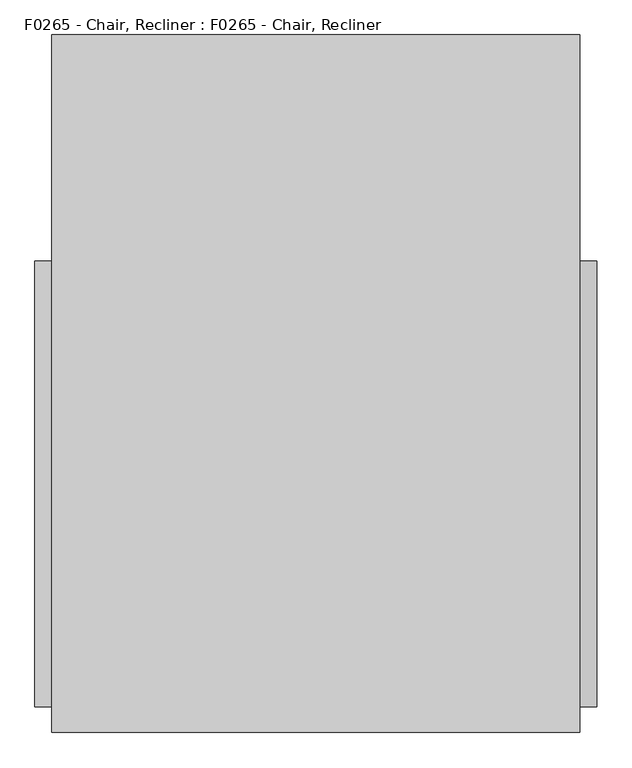
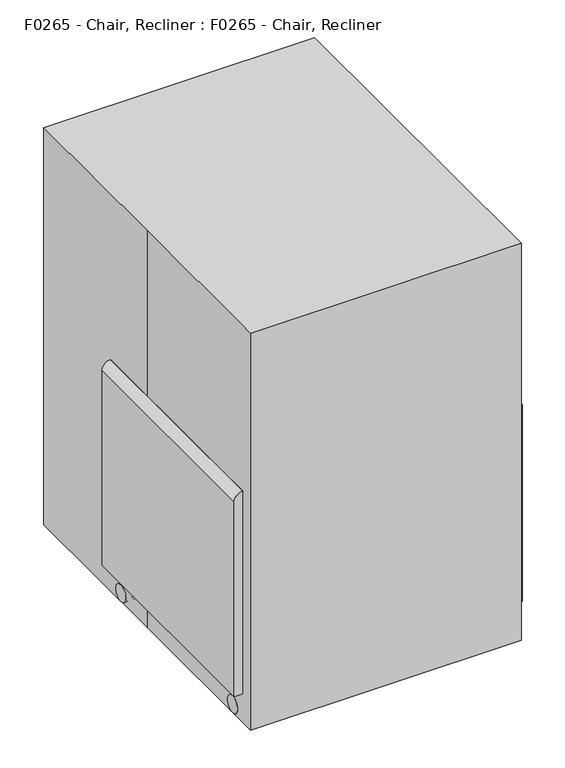
"""IFC4 building model written with IfcOpenShell, lengths in millimetres: proxy geometry, F0265 - Chair, Recliner : F0265 - Chair, Recliner."""

from ifc_helpers import new_model, si_unit, point, frame, frame_2d, origin, origin_with_axes, place, context, project, spatial, polyline, circle_curve, trimmed, segment, composite_curve, outline, extrude, source, transform, mapped, element, save


def f0265_chair_recliner_f0265_chair_recliner_6c0222d9(model_context):
    return source(origin(), model_context, "Body", "SweptSolid", [
        extrude(outline(composite_curve([segment(trimmed(circle_curve(frame_2d((131.7625, 25.4)), 25.4), [point((106.3625, 25.4))], [point((157.1625, 25.4))], False, "CARTESIAN"), True, "CONTINUOUS"), segment(trimmed(circle_curve(frame_2d((131.7625, 25.4)), 25.4), [point((157.1625, 25.4))], [point((106.3625, 25.4))], False, "CARTESIAN"), True, "CONTINUOUS")], self_intersect=False)), frame((-365.125, 0.0, 0.0), z_axis=(1.0, 0.0, 0.0), x_axis=(0.0, 1.0, 0.0)), (0.0, 0.0, 1.0), 9.525),
        extrude(outline(composite_curve([segment(trimmed(circle_curve(frame_2d((-374.65, 141.2875)), 7.9375), [point((-366.7125, 141.2875))], [point((-382.5875, 141.2875))], False, "CARTESIAN"), True, "CONTINUOUS"), segment(trimmed(circle_curve(frame_2d((-374.65, 141.2875)), 7.9375), [point((-382.5875, 141.2875))], [point((-366.7125, 141.2875))], False, "CARTESIAN"), True, "CONTINUOUS")], self_intersect=False)), frame((0.0, 0.0, 24.4243927), z_axis=(0.0, 0.0, 1.0), x_axis=(1.0, 0.0, 0.0)), (0.0, 0.0, 1.0), 64.4756073),
        extrude(outline(composite_curve([segment(trimmed(circle_curve(frame_2d((131.7625, 25.4)), 19.05), [point((150.8125, 25.4))], [point((112.7125, 25.4))], False, "CARTESIAN"), True, "CONTINUOUS"), segment(trimmed(circle_curve(frame_2d((131.7625, 25.4)), 19.05), [point((112.7125, 25.4))], [point((150.8125, 25.4))], False, "CARTESIAN"), True, "CONTINUOUS")], self_intersect=False)), frame((-384.175, 0.0, 0.0), z_axis=(1.0, 0.0, 0.0), x_axis=(0.0, 1.0, 0.0)), (0.0, 0.0, 1.0), 19.05),
        extrude(outline(composite_curve([segment(trimmed(circle_curve(frame_2d((131.7625, 25.4)), 25.4), [point((106.3625, 25.4))], [point((157.1625, 25.4))], False, "CARTESIAN"), True, "CONTINUOUS"), segment(trimmed(circle_curve(frame_2d((131.7625, 25.4)), 25.4), [point((157.1625, 25.4))], [point((106.3625, 25.4))], False, "CARTESIAN"), True, "CONTINUOUS")], self_intersect=False)), frame((-393.7, 0.0, 0.0), z_axis=(1.0, 0.0, 0.0), x_axis=(0.0, 1.0, 0.0)), (0.0, 0.0, 1.0), 9.525),
        extrude(outline(composite_curve([segment(trimmed(circle_curve(frame_2d((131.7625, 25.4)), 25.4), [point((106.3625, 25.4))], [point((157.1625, 25.4))], False, "CARTESIAN"), True, "CONTINUOUS"), segment(trimmed(circle_curve(frame_2d((131.7625, 25.4)), 25.4), [point((157.1625, 25.4))], [point((106.3625, 25.4))], False, "CARTESIAN"), True, "CONTINUOUS")], self_intersect=False)), frame((355.6, 0.0, 0.0), z_axis=(1.0, 0.0, 0.0), x_axis=(0.0, 1.0, 0.0)), (0.0, 0.0, 1.0), 9.525),
        extrude(outline(composite_curve([segment(trimmed(circle_curve(frame_2d((374.65, 141.2875)), 7.9375), [point((366.7125, 141.2875))], [point((382.5875, 141.2875))], False, "CARTESIAN"), True, "CONTINUOUS"), segment(trimmed(circle_curve(frame_2d((374.65, 141.2875)), 7.9375), [point((382.5875, 141.2875))], [point((366.7125, 141.2875))], False, "CARTESIAN"), True, "CONTINUOUS")], self_intersect=False)), frame((0.0, 0.0, 24.4243927), z_axis=(0.0, 0.0, 1.0), x_axis=(1.0, 0.0, 0.0)), (0.0, 0.0, 1.0), 64.4756073),
        extrude(outline(composite_curve([segment(trimmed(circle_curve(frame_2d((131.7625, 25.4)), 19.05), [point((150.8125, 25.4))], [point((112.7125, 25.4))], False, "CARTESIAN"), True, "CONTINUOUS"), segment(trimmed(circle_curve(frame_2d((131.7625, 25.4)), 19.05), [point((112.7125, 25.4))], [point((150.8125, 25.4))], False, "CARTESIAN"), True, "CONTINUOUS")], self_intersect=False)), frame((365.125, 0.0, 0.0), z_axis=(1.0, 0.0, 0.0), x_axis=(0.0, 1.0, 0.0)), (0.0, 0.0, 1.0), 19.05),
        extrude(outline(composite_curve([segment(trimmed(circle_curve(frame_2d((131.7625, 25.4)), 25.4), [point((106.3625, 25.4))], [point((157.1625, 25.4))], False, "CARTESIAN"), True, "CONTINUOUS"), segment(trimmed(circle_curve(frame_2d((131.7625, 25.4)), 25.4), [point((157.1625, 25.4))], [point((106.3625, 25.4))], False, "CARTESIAN"), True, "CONTINUOUS")], self_intersect=False)), frame((384.175, 0.0, 0.0), z_axis=(1.0, 0.0, 0.0), x_axis=(0.0, 1.0, 0.0)), (0.0, 0.0, 1.0), 9.525),
        extrude(outline(composite_curve([segment(trimmed(circle_curve(frame_2d((-430.2125, 25.4)), 25.4), [point((-404.8125, 25.4))], [point((-455.6125, 25.4))], False, "CARTESIAN"), True, "CONTINUOUS"), segment(trimmed(circle_curve(frame_2d((-430.2125, 25.4)), 25.4), [point((-455.6125, 25.4))], [point((-404.8125, 25.4))], False, "CARTESIAN"), True, "CONTINUOUS")], self_intersect=False)), frame((-365.125, 0.0, 0.0), z_axis=(1.0, 0.0, 0.0), x_axis=(0.0, 1.0, 0.0)), (0.0, 0.0, 1.0), 9.525),
        extrude(outline(composite_curve([segment(trimmed(circle_curve(frame_2d((-374.65, -439.7375)), 7.9375), [point((-366.7125, -439.7375))], [point((-382.5875, -439.7375))], False, "CARTESIAN"), True, "CONTINUOUS"), segment(trimmed(circle_curve(frame_2d((-374.65, -439.7375)), 7.9375), [point((-382.5875, -439.7375))], [point((-366.7125, -439.7375))], False, "CARTESIAN"), True, "CONTINUOUS")], self_intersect=False)), frame((0.0, 0.0, 24.4243927), z_axis=(0.0, 0.0, 1.0), x_axis=(1.0, 0.0, 0.0)), (0.0, 0.0, 1.0), 64.4756073),
        extrude(outline(composite_curve([segment(trimmed(circle_curve(frame_2d((-430.2125, 25.4)), 19.05), [point((-449.2625, 25.4))], [point((-411.1625, 25.4))], False, "CARTESIAN"), True, "CONTINUOUS"), segment(trimmed(circle_curve(frame_2d((-430.2125, 25.4)), 19.05), [point((-411.1625, 25.4))], [point((-449.2625, 25.4))], False, "CARTESIAN"), True, "CONTINUOUS")], self_intersect=False)), frame((-384.175, 0.0, 0.0), z_axis=(1.0, 0.0, 0.0), x_axis=(0.0, 1.0, 0.0)), (0.0, 0.0, 1.0), 19.05),
        extrude(outline(composite_curve([segment(trimmed(circle_curve(frame_2d((-430.2125, 25.4)), 25.4), [point((-404.8125, 25.4))], [point((-455.6125, 25.4))], False, "CARTESIAN"), True, "CONTINUOUS"), segment(trimmed(circle_curve(frame_2d((-430.2125, 25.4)), 25.4), [point((-455.6125, 25.4))], [point((-404.8125, 25.4))], False, "CARTESIAN"), True, "CONTINUOUS")], self_intersect=False)), frame((-393.7, 0.0, 0.0), z_axis=(1.0, 0.0, 0.0), x_axis=(0.0, 1.0, 0.0)), (0.0, 0.0, 1.0), 9.525),
        extrude(outline(composite_curve([segment(trimmed(circle_curve(frame_2d((-430.2125, 25.4)), 25.4), [point((-404.8125, 25.4))], [point((-455.6125, 25.4))], False, "CARTESIAN"), True, "CONTINUOUS"), segment(trimmed(circle_curve(frame_2d((-430.2125, 25.4)), 25.4), [point((-455.6125, 25.4))], [point((-404.8125, 25.4))], False, "CARTESIAN"), True, "CONTINUOUS")], self_intersect=False)), frame((355.6, 0.0, 0.0), z_axis=(1.0, 0.0, 0.0), x_axis=(0.0, 1.0, 0.0)), (0.0, 0.0, 1.0), 9.525),
        extrude(outline(composite_curve([segment(trimmed(circle_curve(frame_2d((374.65, -439.7375)), 7.9375), [point((366.7125, -439.7375))], [point((382.5875, -439.7375))], False, "CARTESIAN"), True, "CONTINUOUS"), segment(trimmed(circle_curve(frame_2d((374.65, -439.7375)), 7.9375), [point((382.5875, -439.7375))], [point((366.7125, -439.7375))], False, "CARTESIAN"), True, "CONTINUOUS")], self_intersect=False)), frame((0.0, 0.0, 24.4243927), z_axis=(0.0, 0.0, 1.0), x_axis=(1.0, 0.0, 0.0)), (0.0, 0.0, 1.0), 64.4756073),
        extrude(outline(composite_curve([segment(trimmed(circle_curve(frame_2d((-430.2125, 25.4)), 19.05), [point((-449.2625, 25.4))], [point((-411.1625, 25.4))], False, "CARTESIAN"), True, "CONTINUOUS"), segment(trimmed(circle_curve(frame_2d((-430.2125, 25.4)), 19.05), [point((-411.1625, 25.4))], [point((-449.2625, 25.4))], False, "CARTESIAN"), True, "CONTINUOUS")], self_intersect=False)), frame((365.125, 0.0, 0.0), z_axis=(1.0, 0.0, 0.0), x_axis=(0.0, 1.0, 0.0)), (0.0, 0.0, 1.0), 19.05),
        extrude(outline(composite_curve([segment(trimmed(circle_curve(frame_2d((-430.2125, 25.4)), 25.4), [point((-404.8125, 25.4))], [point((-455.6125, 25.4))], False, "CARTESIAN"), True, "CONTINUOUS"), segment(trimmed(circle_curve(frame_2d((-430.2125, 25.4)), 25.4), [point((-455.6125, 25.4))], [point((-404.8125, 25.4))], False, "CARTESIAN"), True, "CONTINUOUS")], self_intersect=False)), frame((384.175, 0.0, 0.0), z_axis=(1.0, 0.0, 0.0), x_axis=(0.0, 1.0, 0.0)), (0.0, 0.0, 1.0), 9.525),
        extrude(outline(polyline([(330.2, 182.829858), (330.2, 132.029858), (-330.2, 132.029858), (-330.2, 182.829858), (330.2, 182.829858)])), frame((0.0, 0.0, 88.9), z_axis=(0.0, 0.0, 1.0), x_axis=(1.0, 0.0, 0.0)), (0.0, 0.0, 1.0), 330.2),
        extrude(outline(composite_curve([segment(polyline([(111.703548, 399.3779888), (62.634516, 412.5259963)]), True, "CONTINUOUS"), segment(trimmed(circle_curve(frame_2d((69.2085197, 437.0605122)), 25.4), [point((62.634516, 412.5259963))], [point((44.6740037, 443.634516))], False, "CARTESIAN"), True, "CONTINUOUS"), segment(polyline([(44.6740037, 443.634516), (235.8233241, 1157.0134915)]), True, "CONTINUOUS"), segment(trimmed(circle_curve(frame_2d((260.3578401, 1150.4394878)), 25.4), [point((235.8233241, 1157.0134915))], [point((266.9318439, 1174.9740037))], False, "CARTESIAN"), True, "CONTINUOUS"), segment(polyline([(266.9318439, 1174.9740037), (316.0008758, 1161.8259963)]), True, "CONTINUOUS"), segment(trimmed(circle_curve(frame_2d((309.4268721, 1137.2914803)), 25.4), [point((316.0008758, 1161.8259963))], [point((333.9613881, 1130.7174765))], False, "CARTESIAN"), True, "CONTINUOUS"), segment(polyline([(333.9613881, 1130.7174765), (142.8120677, 417.338501)]), True, "CONTINUOUS"), segment(trimmed(circle_curve(frame_2d((118.2775517, 423.9125048)), 25.4), [point((142.8120677, 417.338501))], [point((111.703548, 399.3779888))], False, "CARTESIAN"), True, "CONTINUOUS")], self_intersect=False)), frame((-330.2, 0.0, 0.0), z_axis=(1.0, 0.0, 0.0), x_axis=(0.0, 1.0, 0.0)), (0.0, 0.0, 1.0), 660.4),
        extrude(outline(composite_curve([segment(polyline([(711.2, -355.6), (711.2, -393.7)]), True, "CONTINUOUS"), segment(trimmed(circle_curve(frame_2d((685.8, -393.7)), 25.4), [point((711.2, -393.7))], [point((685.8, -419.1))], False, "CARTESIAN"), True, "CONTINUOUS"), segment(polyline([(685.8, -419.1), (88.9, -419.1), (88.9, -330.2), (685.8, -330.2)]), True, "CONTINUOUS"), segment(trimmed(circle_curve(frame_2d((685.8, -355.6)), 25.4), [point((685.8, -330.2))], [point((711.2, -355.6))], False, "CARTESIAN"), True, "CONTINUOUS")], self_intersect=False)), frame((0.0, -482.6, 0.0), z_axis=(0.0, 1.0, 0.0), x_axis=(0.0, 0.0, 1.0)), (0.0, 0.0, 1.0), 665.429858),
        extrude(outline(composite_curve([segment(polyline([(711.2, 393.7), (711.2, 355.6)]), True, "CONTINUOUS"), segment(trimmed(circle_curve(frame_2d((685.8, 355.6)), 25.4), [point((711.2, 355.6))], [point((685.8, 330.2))], False, "CARTESIAN"), True, "CONTINUOUS"), segment(polyline([(685.8, 330.2), (88.9, 330.2), (88.9, 419.1), (685.8, 419.1)]), True, "CONTINUOUS"), segment(trimmed(circle_curve(frame_2d((685.8, 393.7)), 25.4), [point((685.8, 419.1))], [point((711.2, 393.7))], False, "CARTESIAN"), True, "CONTINUOUS")], self_intersect=False)), frame((0.0, -482.6, 0.0), z_axis=(0.0, 1.0, 0.0), x_axis=(0.0, 0.0, 1.0)), (0.0, 0.0, 1.0), 665.429858),
        extrude(outline(composite_curve([segment(polyline([(406.4, 269.6121072), (406.4, -266.7)]), True, "CONTINUOUS"), segment(trimmed(circle_curve(frame_2d((355.6, -266.7)), 50.8), [point((406.4, -266.7))], [point((355.6, -317.5))], False, "CARTESIAN"), True, "CONTINUOUS"), segment(polyline([(355.6, -317.5), (139.7, -317.5)]), True, "CONTINUOUS"), segment(trimmed(circle_curve(frame_2d((139.7, -266.7)), 50.8), [point((139.7, -317.5))], [point((88.9, -266.7))], False, "CARTESIAN"), True, "CONTINUOUS"), segment(polyline([(88.9, -266.7), (88.9, 269.6121072)]), True, "CONTINUOUS"), segment(trimmed(circle_curve(frame_2d((139.7, 269.6121072)), 50.8), [point((88.9, 269.6121072))], [point((139.7, 320.4121072))], False, "CARTESIAN"), True, "CONTINUOUS"), segment(polyline([(139.7, 320.4121072), (355.6, 320.4121072)]), True, "CONTINUOUS"), segment(trimmed(circle_curve(frame_2d((355.6, 269.6121072)), 50.8), [point((355.6, 320.4121072))], [point((406.4, 269.6121072))], False, "CARTESIAN"), True, "CONTINUOUS")], self_intersect=False)), frame((0.0, -482.6, 0.0), z_axis=(0.0, 1.0, 0.0), x_axis=(0.0, 0.0, 1.0)), (0.0, 0.0, 1.0), 101.6),
        extrude(outline(composite_curve([segment(trimmed(circle_curve(frame_2d((279.4, -12.7)), 50.8), [point((279.4, 38.1))], [point((330.2, -12.7))], False, "CARTESIAN"), True, "CONTINUOUS"), segment(polyline([(330.2, -12.7), (330.2, -431.8)]), True, "CONTINUOUS"), segment(trimmed(circle_curve(frame_2d((279.4, -431.8)), 50.8), [point((330.2, -431.8))], [point((279.4, -482.6))], False, "CARTESIAN"), True, "CONTINUOUS"), segment(polyline([(279.4, -482.6), (-279.4, -482.6)]), True, "CONTINUOUS"), segment(trimmed(circle_curve(frame_2d((-279.4, -431.8)), 50.8), [point((-279.4, -482.6))], [point((-330.2, -431.8))], False, "CARTESIAN"), True, "CONTINUOUS"), segment(polyline([(-330.2, -431.8), (-330.2, -12.7)]), True, "CONTINUOUS"), segment(trimmed(circle_curve(frame_2d((-279.4, -12.7)), 50.8), [point((-330.2, -12.7))], [point((-279.4, 38.1))], False, "CARTESIAN"), True, "CONTINUOUS"), segment(polyline([(-279.4, 38.1), (279.4, 38.1)]), True, "CONTINUOUS")], self_intersect=False)), frame((0.0, 0.0, 419.1), z_axis=(0.0, 0.0, 1.0), x_axis=(1.0, 0.0, 0.0)), (0.0, 0.0, 1.0), 101.6),
        extrude(outline(polyline([(-393.7, 520.7), (393.7, 520.7), (393.7, -520.7), (-393.7, -520.7), (-393.7, 0.0), (-393.7, 520.7)])), origin_with_axes(), (0.0, 0.0, 1.0), 1219.2),
    ])


if __name__ == "__main__":
    model = new_model("IFC4")
    model_context = context("Model", 3, world=origin())
    ifc_project = project(units=[si_unit("LENGTHUNIT", "METRE", prefix="MILLI")], contexts=[model_context])
    site = spatial("IfcSite", under=ifc_project)
    building = spatial("IfcBuilding", under=site)
    placement = place(None, origin())
    f0265_chair_recliner_f0265_chair_recliner_shape = f0265_chair_recliner_f0265_chair_recliner_6c0222d9(model_context)
    element("IfcBuildingElementProxy", 1, Name="F0265 - Chair, Recliner : F0265 - Chair, Recliner", ObjectType="F0265 - Chair, Recliner : F0265 - Chair, Recliner", at=placement, inside=building, context=model_context, shape_type="MappedRepresentation", body=[
        mapped(f0265_chair_recliner_f0265_chair_recliner_shape, transform((0.0, 0.0, 0.0), x_axis=(1.0, 0.0, 0.0), y_axis=(0.0, 1.0, 0.0), z_axis=(0.0, 0.0, 1.0))),
    ])
    save(model, "model.ifc")

# Revit data of these elements
# Type "F0265 - Chair, Recliner : F0265 - Chair, Recliner"
#   Watts2 = "0"
#   Watts1 = "0"
#   Unit_Issue = "EA"
#   UTIL_6_Misc = "-"
#   UTIL_5_NonMedGas = "-"
#   UTIL_4_MiscGas = "-"
#   UTIL_3_MedGas = "-"
#   UTIL_2_Elec = "-"
#   UTIL_1_WaterDrain = "-"
#   Nomenclature = "Chair, Recliner"
#   NSN = "6530"
#   Location [instance default] = ""
#   JSN = "F0265"
#   Fund_Source_VA = "-"
#   Fund_Source_Navy = "-"
#   Fund_Source_Army = "-"
#   Fund_Source_AF = "-"
#   ELEC_Volts2 = "0"
#   ELEC_Volts1 = "0"
#   ELEC_Phase2 = "0"
#   ELEC_Phase1 = "0"
#   ELEC_HertzSwitch = "0"
#   ELEC_HertzDependent = "0"
#   ELEC_Hertz = "0"
#   ELEC_Amps2 = "0"
#   ELEC_Amps1 = "0"
#   DetailDescription = "Reclining chair, 46\" high X 33\" wide X 40\"deep with arms, straight leg base and floor glides or lockable two (2) inch casters. Seat, back and foot rest are foam padded and upholstered with woven textile fabric or vinyl."
#   CAT_VA = "C"
#   CAT_Navy = "C"
#   CAT_IHS = "-"
#   CAT_Army = "C"
#   CAT_AF = "C"
#   BTUperhour = "0"
#   radius = 0' - 1"
#   calc 2 = 0' - 0.33333"
#   calc 1 = 0' - 0.66667"
#   Weight_IP = 131
#   DIM_Width_IP = 2' - 7"
#   DIM_Height_IP = 4' - 0"
#   DIM_Depth_IP = 3' - 5"
#   finish [instance default] = none
# Element 1 (IfcBuildingElementProxy, "F0265 - Chair, Recliner : F0265 - Chair, Recliner")
#   Location = "LDAT2"
#   Materials on its faces: "EquipSpace"
# Materials
#   "EquipSpace": class "Unassigned", colour RGB 221 217 195, transparency 0.5
